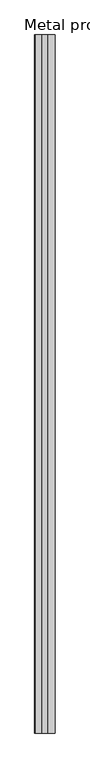
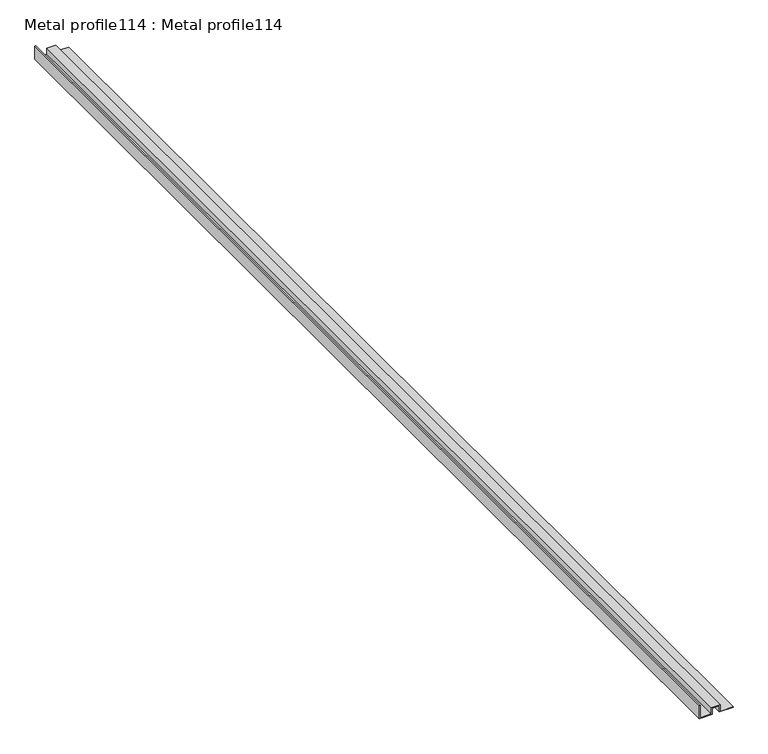
"""IFC4 building model written with IfcOpenShell, lengths in millimetres: proxy geometry, Metal profile114 : Metal profile114."""

from ifc_helpers import new_model, si_unit, frame, origin, place, context, project, spatial, polyline, outline, extrude, source, transform, mapped, element, save


def metal_profile114_metal_profile114_e97886af(model_context):
    return source(origin(), model_context, "Body", "SweptSolid", [
        extrude(outline(polyline([(39540.7420603, -2790.7255764), (39540.7420603, -2768.5005764), (39552.1720603, -2768.5005764), (39552.1720603, -2755.8005764), (39540.7420603, -2755.8005764), (39540.7420603, -2732.0873925), (39542.0220603, -2732.0873925), (39542.0220603, -2754.5205764), (39553.4520603, -2754.5205764), (39553.4520603, -2769.7805764), (39542.0220603, -2769.7805764), (39542.0220603, -2789.4455764), (39564.5428218, -2789.4455764), (39564.5428218, -2790.7255764), (39540.7420603, -2790.7255764)])), frame((0.0, 999.7499999, 0.0), z_axis=(0.0, 1.0, 0.0), x_axis=(0.0, 0.0, 1.0)), (0.0, 0.0, 1.0), 2000.0),
    ])


if __name__ == "__main__":
    model = new_model("IFC4")
    model_context = context("Model", 3, world=origin())
    ifc_project = project(units=[si_unit("LENGTHUNIT", "METRE", prefix="MILLI")], contexts=[model_context])
    site = spatial("IfcSite", under=ifc_project)
    building = spatial("IfcBuilding", under=site)
    placement = place(None, origin())
    metal_profile114_metal_profile114_shape = metal_profile114_metal_profile114_e97886af(model_context)
    element("IfcBuildingElementProxy", 1, Name="Metal profile114 : Metal profile114", ObjectType="Metal profile114 : Metal profile114", at=placement, inside=building, context=model_context, shape_type="MappedRepresentation", body=[
        mapped(metal_profile114_metal_profile114_shape, transform((0.0, 0.0, 0.0), x_axis=(1.0, 0.0, 0.0), y_axis=(0.0, 1.0, 0.0), z_axis=(0.0, 0.0, 1.0))),
    ])
    save(model, "model.ifc")

# Revit data of these elements
# Type "Metal profile114 : Metal profile114"
#   NameOverride = "Metal profile114"
# Element 1 (IfcBuildingElementProxy, "Metal profile114 : Metal profile114")
#   Materials on its faces: "16 GA. COPPER SOFFIT DRIP SCREED"
# Materials
#   "16 GA. COPPER SOFFIT DRIP SCREED": class "Unassigned", colour RGB 255 217 0, transparency 0
